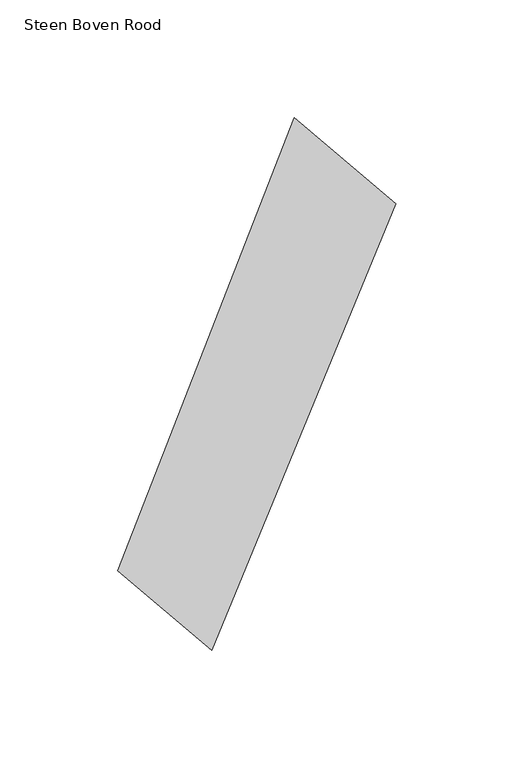
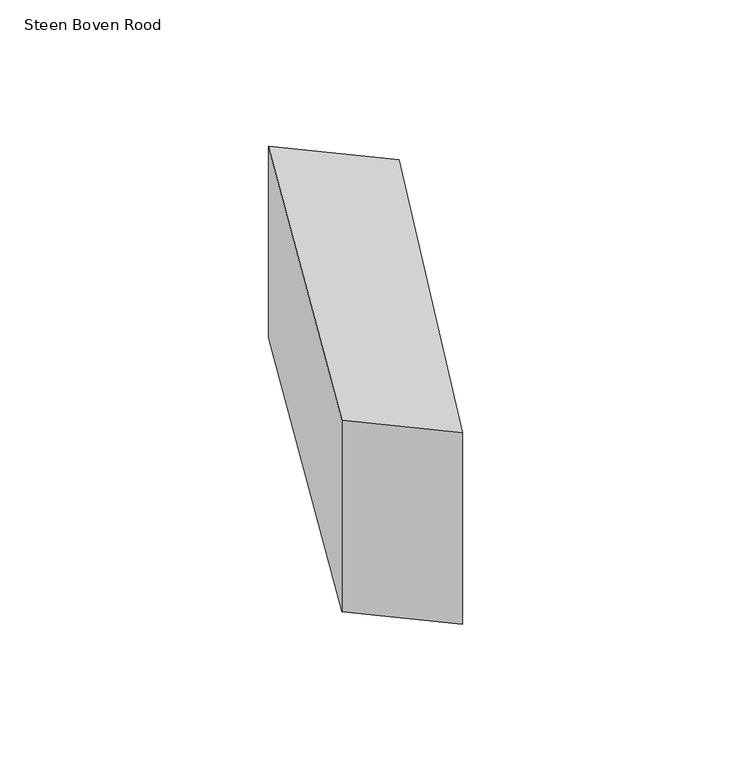
"""IFC4 building model written with IfcOpenShell, lengths in millimetres: proxy geometry, 00_GMA_steen_versie_4 : Steen Boven Rood."""

from ifc_helpers import new_model, si_unit, origin, origin_with_axes, place, context, project, spatial, polyline, outline, extrude, source, transform, mapped, element, save


def steen_boven_rood_4c230b22(model_context):
    return source(origin(), model_context, "Body", "SweptSolid", [
        extrude(outline(polyline([(141.812267, 168.9495187), (63.5707465, -20.6713609), (23.6423327, 13.1339685), (98.582844, 205.5873147), (141.812267, 168.9495187)])), origin_with_axes(), (0.0, 0.0, 1.0), 100.0),
    ])


if __name__ == "__main__":
    model = new_model("IFC4")
    model_context = context("Model", 3, world=origin())
    ifc_project = project(units=[si_unit("LENGTHUNIT", "METRE", prefix="MILLI")], contexts=[model_context])
    site = spatial("IfcSite", under=ifc_project)
    building = spatial("IfcBuilding", under=site)
    placement = place(None, origin())
    steen_boven_rood_shape = steen_boven_rood_4c230b22(model_context)
    element("IfcBuildingElementProxy", 1, Name="00_GMA_steen_versie_4 : Steen Boven Rood", ObjectType="00_GMA_steen_versie_4 : Steen Boven Rood", at=placement, inside=building, context=model_context, shape_type="MappedRepresentation", body=[
        mapped(steen_boven_rood_shape, transform((0.0, 0.0, 0.0), x_axis=(1.0, 0.0, 0.0), y_axis=(0.0, 1.0, 0.0), z_axis=(0.0, 0.0, 1.0))),
    ])
    save(model, "model.ifc")

# Revit data of these elements
# Type "00_GMA_steen_versie_4 : Steen Boven Rood"
#   StootVoegHalfBoven [instance default] = 5 mm
#   StootVoegHalf [instance default] = 5 mm
#   StootVoegBreedteOnder = 10 mm
#   StootVoegBreedteBoven = 10 mm
#   Steendikte = 100 mm
#   LintVoegOnderHalf = 5 mm
#   LintVoegOnder = 10 mm
#   LintVoegBovenHalf = 0 mm
#   LintVoegBoven = 0 mm
#   materiaal = 21_steen_rood
#   MateriaalVoeg = none
#   Default Elevation = 0
# Element 1 (IfcBuildingElementProxy, "00_GMA_steen_versie_4 : Steen Boven Rood")
#   Materials on its faces: "21_steen_rood"
# Materials
#   "21_steen_rood": class "Unassigned", colour RGB 213 111 43, transparency 0, Cost = 0
